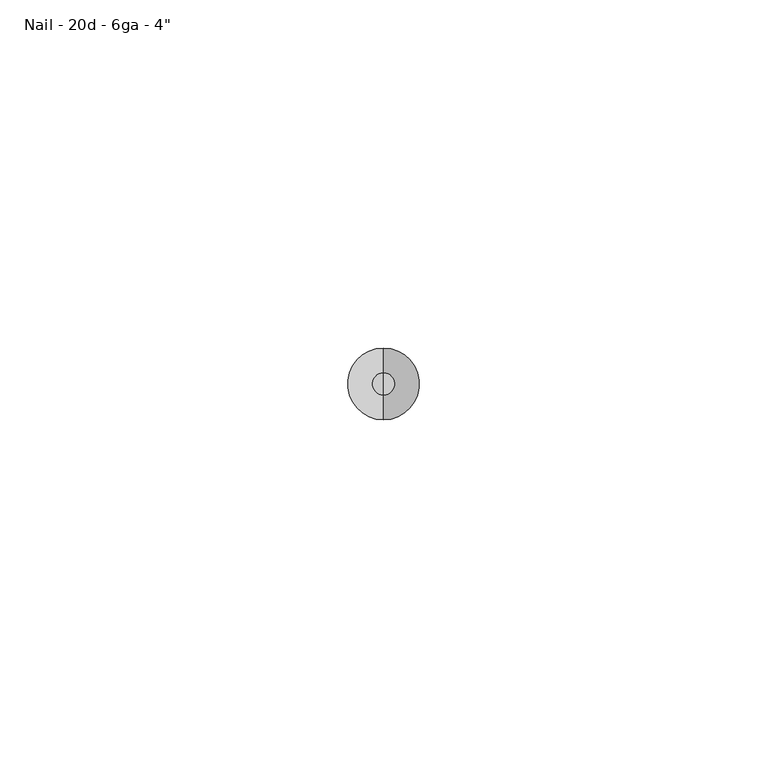
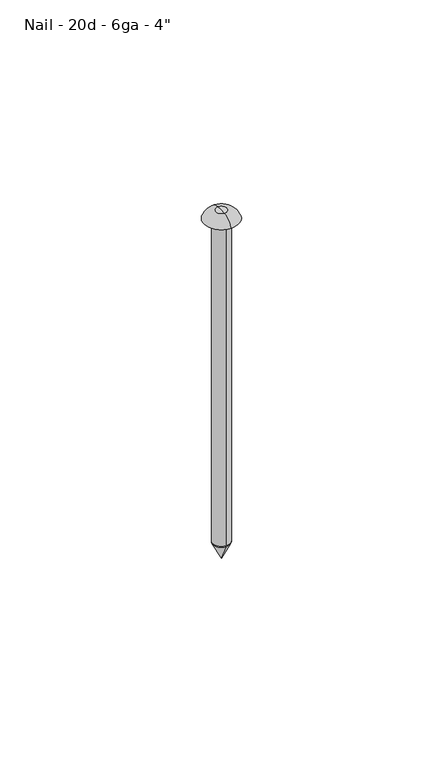
"""IFC4 building model written with IfcOpenShell, lengths in millimetres: fastener geometry."""

from ifc_helpers import new_model, si_unit, point, frame, origin, origin_2d, place, context, project, spatial, polyline, circle_curve, ellipse_curve, trimmed, segment, composite_curve, outline, extrude, source, transform, mapped, element, save
from ifc_brep_helpers import plane_surface, revolved_surface, advanced_brep


def fastener_621c100d(model_context):
    return source(origin(), model_context, "Body", "SolidModel", [
        advanced_brep(
        [(0.0, -2.5781, -101.6), (0.0, 2.5781, -101.6), (0.0, 0.0, -101.6), (0.0, 0.0, -106.7562)],
        [
            (0, 1, circle_curve(frame((0.0, 0.0, -101.6), z_axis=(0.0, 0.0, 1.0), x_axis=(0.0, 1.0, 0.0)), 2.5781)),
            (1, 2),
            (2, 0),
            (1, 0, circle_curve(frame((0.0, 0.0, -101.6), z_axis=(0.0, 0.0, 1.0), x_axis=(0.0, 1.0, 0.0)), 2.5781)),
            (3, 1),
            (0, 3),
        ],
        [
            plane_surface(frame((0.0, 0.0, -101.6), z_axis=(0.0, 0.0, 1.0), x_axis=(0.0, 1.0, 0.0))),
            revolved_surface(polyline([(0.0, 2.5781, -101.6), (0.0, 0.0, -106.7562)]), (0.0, 0.0, -103.0840259), (0.0, 0.0, -1.0)),
        ],
        [
            (0, [[1, 2, 3]]),
            (0, [[4, -3, -2]]),
            (1, [[5, -1, 6]]),
            (1, [[-6, -4, -5]]),
        ],
    ),
        advanced_brep(
        [(0.0, 5.1562, 0.0), (0.0, -5.1562, 0.0), (0.0, 0.0, 0.0), (0.0, 0.0, 2.5781), (0.0, -1.5875, 2.5781), (0.0, 1.5875, 2.5781)],
        [
            (0, 1, circle_curve(frame((0.0, 0.0, 0.0), z_axis=(0.0, 0.0, -1.0), x_axis=(0.0, -1.0, 0.0)), 5.1562)),
            (1, 2),
            (2, 0),
            (1, 0, circle_curve(frame((0.0, 0.0, 0.0), z_axis=(0.0, 0.0, -1.0), x_axis=(0.0, -1.0, 0.0)), 5.1562)),
            (3, 4),
            (4, 5, circle_curve(frame((0.0, 0.0, 2.5781), z_axis=(0.0, 0.0, 1.0), x_axis=(0.0, -1.0, 0.0)), 1.5875)),
            (5, 3),
            (5, 4, circle_curve(frame((0.0, 0.0, 2.5781), z_axis=(0.0, 0.0, 1.0), x_axis=(0.0, -1.0, 0.0)), 1.5875)),
            (4, 1, circle_curve(frame((0.0, -1.5875, -1.1809123), z_axis=(1.0, 0.0, 0.0), x_axis=(0.0, -1.0, 0.0)), 3.7590123)),
            (0, 5, circle_curve(frame((0.0, 1.5875, -1.1809123), z_axis=(1.0, 0.0, 0.0), x_axis=(0.0, 1.0, 0.0)), 3.7590123)),
        ],
        [
            plane_surface(frame((0.0, 0.0, 0.0), z_axis=(0.0, 0.0, -1.0), x_axis=(0.0, -1.0, 0.0))),
            plane_surface(frame((0.0, 0.0, 2.5781), z_axis=(0.0, 0.0, 1.0), x_axis=(0.0, -1.0, 0.0))),
            revolved_surface(trimmed(ellipse_curve(frame((0.0, -1.5875, -1.1809123), z_axis=(-1.0, 0.0, 0.0), x_axis=(0.0, -1.0, 0.0)), 3.7590123, 3.7590123), [point((0.0, -5.1562, 0.0))], [point((0.0, -1.5875, 2.5781))], True, "CARTESIAN"), (0.0, 0.0, 1.4840259), (0.0, 0.0, 1.0)),
        ],
        [
            (0, [[1, 2, 3]]),
            (0, [[4, -3, -2]]),
            (1, [[5, 6, 7]]),
            (1, [[-7, 8, -5]]),
            (2, [[-6, 9, -1, 10]]),
            (2, [[-8, -10, -4, -9]]),
        ],
    ),
        extrude(outline(composite_curve([segment(trimmed(circle_curve(origin_2d(), 2.5781), [point((0.0, -2.5781))], [point((0.0, 2.5781))], False, "CARTESIAN"), True, "CONTINUOUS"), segment(trimmed(circle_curve(origin_2d(), 2.5781), [point((0.0, 2.5781))], [point((0.0, -2.5781))], False, "CARTESIAN"), True, "CONTINUOUS")], self_intersect=False)), frame((0.0, 0.0, -101.6), z_axis=(0.0, 0.0, 1.0), x_axis=(1.0, 0.0, 0.0)), (0.0, 0.0, 1.0), 101.6),
    ])


if __name__ == "__main__":
    model = new_model("IFC4")
    model_context = context("Model", 3, world=origin())
    ifc_project = project(units=[si_unit("LENGTHUNIT", "METRE", prefix="MILLI")], contexts=[model_context])
    site = spatial("IfcSite", under=ifc_project)
    building = spatial("IfcBuilding", under=site)
    placement = place(None, origin())
    fastener_shape = fastener_621c100d(model_context)
    element("IfcFastener", 1, ObjectType="060523 - W_P_C - Fastenings - Generic : Nail - 20d - 6ga - 4\"", at=placement, inside=building, context=model_context, shape_type="MappedRepresentation", body=[
        mapped(fastener_shape, transform((0.0, 0.0, 0.0), x_axis=(1.0, 0.0, 0.0), y_axis=(0.0, 1.0, 0.0), z_axis=(0.0, 0.0, 1.0))),
    ])
    save(model, "model.ifc")

# Revit data of these elements
# Type "060523 - W_P_C - Fastenings - Generic : Nail - 20d - 6ga - 4\""
#   Washer_Thickness = 0' - 0.00333"
#   Washer Radius = 0' - 0.1115"
#   Washer Offset - Head = 0' - 0"
#   Washer Offset = 0' - 0"
#   Thickness_of_Substrate [instance default] = 0' - 1"
#   Side = 0' - 0 37/64"
#   Radius = 0' - 0.1015"
#   Length [instance default] = 0' - 4"
#   Head Size = 0' - 1"
#   Head Radius = 0' - 0 1/2"
#   Head Height = 0' - 0.01"
#   Double Diameter = 0' - 0.406"
#   Diameter = 0' - 0.203"
#   Default Elevation = 4' - 0"
#   Washer_Nut_Visibility = no
#   Washer_Head_Visibility = no
#   Round_Head_Visibility = yes
#   Point Visibility = yes
#   Nut_Visibility = no
#   Hex_Head_Visiblilty = no
#   Washer Material = none
#   Bolt Material (Size) = AT SILL - FASTENER AT 24" O.C.
# Element 1 (IfcFastener, "060523 - W_P_C - Fastenings - Generic : Nail - 20d - 6ga - 4\"")
#   Materials on its faces: "AT SILL - FASTENER AT 24\" O.C."
# Materials
#   "AT SILL - FASTENER AT 24\" O.C.": class "Generic", colour RGB 120 120 120, transparency 0, Cost = 0
